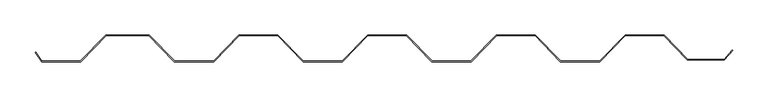
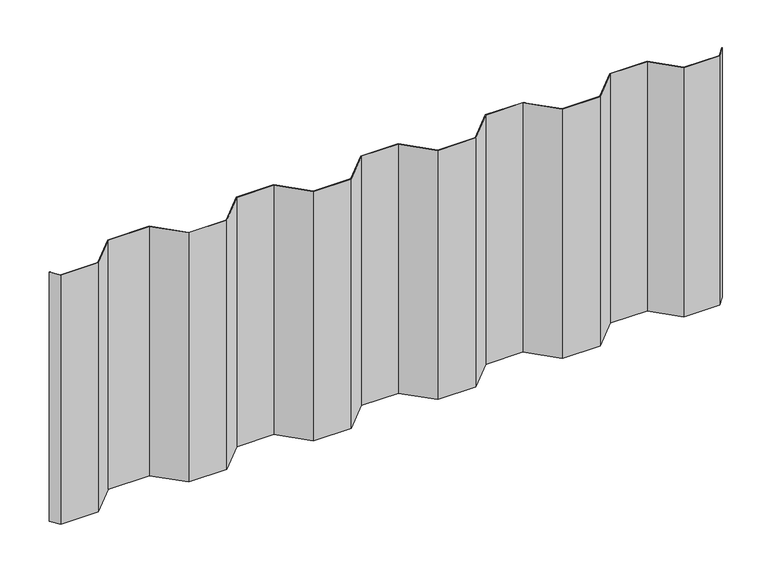
"""IFC4 building model written with IfcOpenShell, lengths in millimetres: proxy geometry, Generic Models 2:Generic Models 2:310765:Generic Models 2:310765 : Generic Models 2:Generic Models 2:310765:3 : Generic Models 2:Generic Models 2:310765:Generic Models 2:310765 : Generic Models 2:Generic Models 2:310765:300385."""

import ifcopenshell
import ifcopenshell.guid

model = None  # the IFC model being written
_history = None  # IfcOwnerHistory: only IFC2X3 demands one
_inside = {}  # id of a spatial element -> (the spatial element, [elements in it])
_under = {}  # id of a project, library or spatial element -> (it, [spatial elements below it])
_declared = {}  # id of a project -> (the project, [libraries it declares])
_typed = {}  # id of a type object -> (the type object, [elements of that type])
_made_of = {}  # id of a material, layer set ... -> (it, [elements and type objects made of it])


def new_model(schema):
    """Start an empty IFC model of exactly this schema.

    Asked for "IFC4X3", IfcOpenShell would pick the latest addendum, in which some entities
    have other attributes; the version numbers below select the first issue.
    IFC2X3 requires an IfcOwnerHistory on every rooted entity: one is made here for all.
    """
    global model, _history
    if schema == "IFC4X3":
        model = ifcopenshell.file(schema_version=(4, 3, 0, 0))
    else:
        model = ifcopenshell.file(schema=schema)
    _inside.clear()
    _under.clear()
    _declared.clear()
    _typed.clear()
    _made_of.clear()
    _history = None
    if model.schema == "IFC2X3":
        org = make("IfcOrganization", Name="unknown")
        user = make(
            "IfcPersonAndOrganization",
            ThePerson=make("IfcPerson", FamilyName="unknown"),
            TheOrganization=org,
        )
        app = make(
            "IfcApplication",
            ApplicationDeveloper=org,
            Version="unknown",
            ApplicationFullName="unknown",
            ApplicationIdentifier="unknown",
        )
        _history = make(
            "IfcOwnerHistory",
            OwningUser=user,
            OwningApplication=app,
            ChangeAction="ADDED",
            CreationDate=0,
        )
    return model


def make(cls, **values):
    """One entity of the class cls with the attributes given. An attribute that is None is left unset."""
    return model.create_entity(
        cls, **{name: value for name, value in values.items() if value is not None}
    )


def rooted(cls, **values):
    """An entity with a GlobalId (a new one), such as an element, a storey or a relation."""
    return make(cls, GlobalId=ifcopenshell.guid.new(), OwnerHistory=_history, **values)


def si_unit(unit_type, name, prefix=None):
    """IfcSIUnit, for example si_unit("LENGTHUNIT", "METRE", prefix="MILLI")."""
    return make("IfcSIUnit", UnitType=unit_type, Prefix=prefix, Name=name)


def assignment(units):
    """IfcUnitAssignment: the units of a project."""
    return None if units is None else make("IfcUnitAssignment", Units=units)


def point(xyz):
    """IfcCartesianPoint."""
    return None if xyz is None else make("IfcCartesianPoint", Coordinates=xyz)


def direction(xyz):
    """IfcDirection."""
    return None if xyz is None else make("IfcDirection", DirectionRatios=xyz)


def frame(location, z_axis=None, x_axis=None):
    """IfcAxis2Placement3D, a coordinate frame: its origin and axes. An axis left out is left unset."""
    return make(
        "IfcAxis2Placement3D",
        Location=point(location),
        Axis=direction(z_axis),
        RefDirection=direction(x_axis),
    )


def origin():
    """The frame at (0, 0, 0) with its axes left unset."""
    return frame((0.0, 0.0, 0.0))


def place(relative_to, where):
    """IfcLocalPlacement: puts the frame where relative to a parent placement (None: the world)."""
    return make(
        "IfcLocalPlacement", PlacementRelTo=relative_to, RelativePlacement=where
    )


def context(
    kind, dimensions, precision=None, world=None, true_north=None, identifier=None
):
    """IfcGeometricRepresentationContext, for example the 3D "Model" context."""
    return make(
        "IfcGeometricRepresentationContext",
        ContextIdentifier=identifier,
        ContextType=kind,
        CoordinateSpaceDimension=dimensions,
        Precision=precision,
        WorldCoordinateSystem=world,
        TrueNorth=true_north,
    )


def project(units=None, contexts=None):
    """IfcProject with its units and contexts."""
    return rooted(
        "IfcProject",
        Name="project",
        RepresentationContexts=contexts,
        UnitsInContext=assignment(units),
    )


def spatial(cls, under=None, at=None, **own):
    """A site, building, storey or space (cls), placed at a placement, below another one or the project."""
    s = rooted(cls, ObjectPlacement=at, **own)
    if under is not None:
        _under.setdefault(under.id(), (under, []))[1].append(s)
    return s


def polyline(points):
    """IfcPolyline through the points."""
    return make("IfcPolyline", Points=[point(p) for p in points])


def outline(outer, holes=None, kind="AREA"):
    """IfcArbitraryClosedProfileDef: a profile drawn as a closed curve; with holes, ...WithVoids."""
    if holes is None:
        return make("IfcArbitraryClosedProfileDef", ProfileType=kind, OuterCurve=outer)
    return make(
        "IfcArbitraryProfileDefWithVoids",
        ProfileType=kind,
        OuterCurve=outer,
        InnerCurves=holes,
    )


def extrude(swept, where, along, depth):
    """IfcExtrudedAreaSolid: the profile swept, set in the frame where, extruded along a direction by depth."""
    return make(
        "IfcExtrudedAreaSolid",
        SweptArea=swept,
        Position=where,
        ExtrudedDirection=direction(along),
        Depth=depth,
    )


def shape(context_of_items, identifier, shape_type, items):
    """IfcShapeRepresentation: the items that make up one representation, for example the "Body"."""
    return make(
        "IfcShapeRepresentation",
        ContextOfItems=context_of_items,
        RepresentationIdentifier=identifier,
        RepresentationType=shape_type,
        Items=items,
    )


def source(mapping_origin, context_of_items, identifier, shape_type, items):
    """IfcRepresentationMap: a shape defined once, which mapped items show again and again."""
    return make(
        "IfcRepresentationMap",
        MappingOrigin=mapping_origin,
        MappedRepresentation=shape(context_of_items, identifier, shape_type, items),
    )


def transform(
    local_origin,
    x_axis=None,
    y_axis=None,
    z_axis=None,
    scale=None,
    scale2=None,
    scale3=None,
    uniform=True,
):
    """IfcCartesianTransformationOperator3D, or its non-uniform kind. x_axis, y_axis, z_axis: its Axis1, 2, 3."""
    if uniform:
        return make(
            "IfcCartesianTransformationOperator3D",
            Axis1=direction(x_axis),
            Axis2=direction(y_axis),
            LocalOrigin=point(local_origin),
            Scale=scale,
            Axis3=direction(z_axis),
        )
    return make(
        "IfcCartesianTransformationOperator3DnonUniform",
        Axis1=direction(x_axis),
        Axis2=direction(y_axis),
        LocalOrigin=point(local_origin),
        Scale=scale,
        Axis3=direction(z_axis),
        Scale2=scale2,
        Scale3=scale3,
    )


def mapped(mapping_source, mapping_target):
    """IfcMappedItem: shows the shape of a source again, moved by a transform."""
    return make(
        "IfcMappedItem", MappingSource=mapping_source, MappingTarget=mapping_target
    )


def made_of(thing, what):
    """Note that an element or type object is made of a material, layer set ...; save() writes the relation."""
    if what is not None:
        _made_of.setdefault(what.id(), (what, []))[1].append(thing)
    return thing


def element(
    cls,
    number,
    at=None,
    inside=None,
    cuts=None,
    type_object=None,
    material=None,
    context=None,
    identifier="Body",
    shape_type=None,
    held_by="IfcProductDefinitionShape",
    body=None,
    shapes=None,
    **own,
):
    """One element of the class cls, such as IfcWall. Its Tag is "e" and its number.

    at: its placement. inside: the storey or other place that contains it. cuts: it is an
    opening in that element (IfcRelVoidsElement). A single representation is given by context,
    identifier, shape_type and body (its items); several are given by shapes. held_by: the class
    of the entity that holds the representations. save() writes the other relations.
    """
    e = rooted(cls, Tag="e%d" % number, ObjectPlacement=at, **own)
    if body is not None:
        shapes = [shape(context, identifier, shape_type, body)]
    if shapes is not None:
        e.Representation = make(held_by, Representations=shapes)
    if inside is not None:
        _inside.setdefault(inside.id(), (inside, []))[1].append(e)
    if cuts is not None:
        rooted(
            "IfcRelVoidsElement", RelatingBuildingElement=cuts, RelatedOpeningElement=e
        )
    if type_object is not None:
        _typed.setdefault(type_object.id(), (type_object, []))[1].append(e)
    return made_of(e, material)


def aggregate(whole, parts):
    """IfcRelAggregates: a whole, such as a stair, and the parts it consists of."""
    return rooted("IfcRelAggregates", RelatingObject=whole, RelatedObjects=parts)


def save(model, path):
    """Write the relations noted so far, then the file.

    IfcRelAggregates (storeys below a building ...), IfcRelContainedInSpatialStructure (elements
    in a storey), IfcRelDefinesByType, IfcRelAssociatesMaterial and IfcRelDeclares: one each for
    every whole, place, type object, material and project.
    """
    for whole, parts in _under.values():
        aggregate(whole, parts)
    for where, things in _inside.values():
        rooted(
            "IfcRelContainedInSpatialStructure",
            RelatedElements=things,
            RelatingStructure=where,
        )
    for kind, things in _typed.values():
        rooted("IfcRelDefinesByType", RelatedObjects=things, RelatingType=kind)
    for what, things in _made_of.values():
        rooted("IfcRelAssociatesMaterial", RelatedObjects=things, RelatingMaterial=what)
    for by, libraries in _declared.values():
        rooted("IfcRelDeclares", RelatingContext=by, RelatedDefinitions=libraries)
    model.write(path)


def generic_models_9448d0f1(model_context):
    return source(origin(), model_context, "Body", "SweptSolid", [
        extrude(outline(polyline([(593719.8809779, -568266.4432213), (593667.2871722, -568266.4432213), (593633.6551875, -568231.8851341), (593579.1467875, -568231.8851341), (593542.9845958, -568269.1913841), (593486.9373791, -568269.1913841), (593450.7751875, -568231.8851341), (593396.2667875, -568231.8851341), (593360.1045958, -568269.1913841), (593304.0573791, -568269.1913841), (593267.8951875, -568231.8851341), (593213.3867875, -568231.8851341), (593177.2245958, -568269.1913841), (593121.1773791, -568269.1913841), (593085.0151875, -568231.8851341), (593030.5067875, -568231.8851341), (592994.3445958, -568269.1913841), (592938.2973791, -568269.1913841), (592902.1351875, -568231.8851341), (592841.2767875, -568231.8851341), (592805.1145958, -568269.1913841), (592749.8367875, -568269.1913841), (592740.6584173, -568256.0833131), (592741.3086193, -568255.6280368), (592750.2499875, -568268.3976341), (592804.7785503, -568268.3976341), (592840.9407419, -568231.0913841), (592902.471233, -568231.0913841), (592938.6334246, -568268.3976341), (592994.0085503, -568268.3976341), (593030.1707419, -568231.0913841), (593085.351233, -568231.0913841), (593121.5134246, -568268.3976341), (593176.8885503, -568268.3976341), (593213.0507419, -568231.0913841), (593268.231233, -568231.0913841), (593304.3934246, -568268.3976341), (593359.7685503, -568268.3976341), (593395.9307419, -568231.0913841), (593451.111233, -568231.0913841), (593487.2734246, -568268.3976341), (593542.6485503, -568268.3976341), (593578.8107419, -568231.0913841), (593633.9903018, -568231.0913841), (593667.6222866, -568265.6494713), (593719.5286406, -568265.6494713), (593731.1747524, -568252.7731785), (593731.7367242, -568253.3351503), (593719.8809779, -568266.4432213)])), frame((0.0, 0.0, 4503.9520442), z_axis=(0.0, 0.0, 1.0), x_axis=(1.0, 0.0, 0.0)), (0.0, 0.0, 1.0), 387.5312455),
    ])


if __name__ == "__main__":
    model = new_model("IFC4")
    model_context = context("Model", 3, world=origin())
    ifc_project = project(units=[si_unit("LENGTHUNIT", "METRE", prefix="MILLI")], contexts=[model_context])
    site = spatial("IfcSite", under=ifc_project)
    building = spatial("IfcBuilding", under=site)
    placement = place(None, origin())
    generic_models_shape = generic_models_9448d0f1(model_context)
    element("IfcBuildingElementProxy", 1, Name="Generic Models 2:Generic Models 2:310765:Generic Models 2:310765 : Generic Models 2:Generic Models 2:310765:3 : Generic Models 2:Generic Models 2:310765:Generic Models 2:310765 : Generic Models 2:Generic Models 2:310765:300385", ObjectType="Generic Models 2:Generic Models 2:310765:Generic Models 2:310765 : Generic Models 2:Generic Models 2:310765:3 : Generic Models 2:Generic Models 2:310765:Generic Models 2:310765 : Generic Models 2:Generic Models 2:310765:300385", at=placement, inside=building, context=model_context, shape_type="MappedRepresentation", body=[
        mapped(generic_models_shape, transform((0.0, 0.0, 0.0), x_axis=(1.0, 0.0, 0.0), y_axis=(0.0, 1.0, 0.0), z_axis=(0.0, 0.0, 1.0))),
    ])
    save(model, "model.ifc")

# Revit data of these elements
# Type "Generic Models 2:Generic Models 2:310765:Generic Models 2:310765 : Generic Models 2:Generic Models 2:310765:3 : Generic Models 2:Generic Models 2:310765:Generic Models 2:310765 : Generic Models 2:Generic Models 2:310765:300385"
#   NameOverride = "Generic Models 2:Generic Models 2:310765:Generic Models 2:310765 : Generic Models 2:Generic Models 2:310765:300385"
#   ObjectTypeOverride = "Generic Models 2:310765 : Generic Models 2:Generic Models 2:310765"
#   Reference = "Generic Models 2"
#   Tag = "300385"
# Element 1 (IfcBuildingElementProxy, "Generic Models 2:Generic Models 2:310765:Generic Models 2:310765 : Generic Models 2:Generic Models 2:310765:3 : Generic Models 2:Generic Models 2:310765:Generic Models 2:310765 : Generic Models 2:Generic Models 2:310765:300385")
#   Materials on its faces: "VERTICAL CORRUGATED METAL PANEL - EXPOSED FASTENERS - (MBCI 7.2 PANEL)"
# Materials
#   "VERTICAL CORRUGATED METAL PANEL - EXPOSED FASTENERS - (MBCI 7.2 PANEL)": class "Generic", colour RGB 120 120 120, transparency 0, Cost = 0
